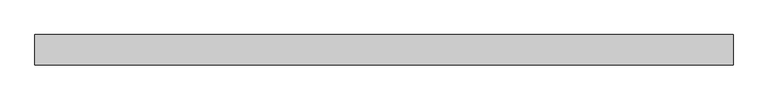
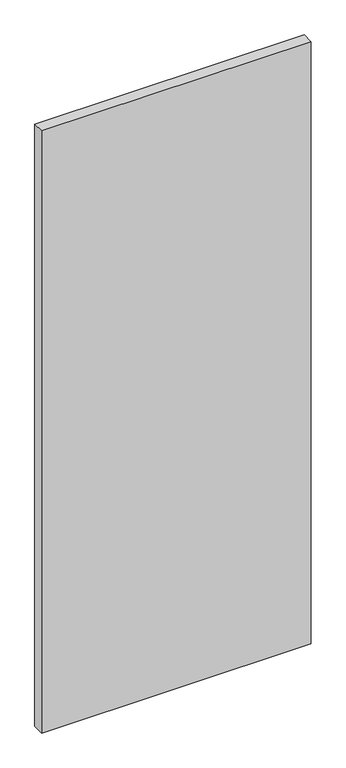
"""IFC4 building model written with IfcOpenShell, lengths in millimetres: proxy geometry, Generic Models 7:Generic Models 1:337419:Generic Models 1:337419 : Generic Models 7:Generic Models 1:337419:50 : Generic Models 7:Generic Models 1:337419:Generic Models 1:337419 : Generic Models 7:Generic Models 1:337419:301336."""

from ifc_helpers import new_model, si_unit, frame, origin, place, context, project, spatial, polyline, outline, extrude, source, transform, mapped, element, save


def generic_models_bfdba70c(model_context):
    return source(origin(), model_context, "Body", "SweptSolid", [
        extrude(outline(polyline([(593738.3225141, -536559.6725858), (593738.3225141, -536604.1225858), (592715.7367242, -536604.1225858), (592715.7367242, -536559.6725858), (593738.3225141, -536559.6725858)])), frame((0.0, 0.0, 22.0396518), z_axis=(0.0, 0.0, 1.0), x_axis=(1.0, 0.0, 0.0)), (0.0, 0.0, 1.0), 2413.3468131),
    ])


if __name__ == "__main__":
    model = new_model("IFC4")
    model_context = context("Model", 3, world=origin())
    ifc_project = project(units=[si_unit("LENGTHUNIT", "METRE", prefix="MILLI")], contexts=[model_context])
    site = spatial("IfcSite", under=ifc_project)
    building = spatial("IfcBuilding", under=site)
    placement = place(None, origin())
    generic_models_shape = generic_models_bfdba70c(model_context)
    element("IfcBuildingElementProxy", 1, Name="Generic Models 7:Generic Models 1:337419:Generic Models 1:337419 : Generic Models 7:Generic Models 1:337419:50 : Generic Models 7:Generic Models 1:337419:Generic Models 1:337419 : Generic Models 7:Generic Models 1:337419:301336", ObjectType="Generic Models 7:Generic Models 1:337419:Generic Models 1:337419 : Generic Models 7:Generic Models 1:337419:50 : Generic Models 7:Generic Models 1:337419:Generic Models 1:337419 : Generic Models 7:Generic Models 1:337419:301336", at=placement, inside=building, context=model_context, shape_type="MappedRepresentation", body=[
        mapped(generic_models_shape, transform((0.0, 0.0, 0.0), x_axis=(1.0, 0.0, 0.0), y_axis=(0.0, 1.0, 0.0), z_axis=(0.0, 0.0, 1.0))),
    ])
    save(model, "model.ifc")

# Revit data of these elements
# Type "Generic Models 7:Generic Models 1:337419:Generic Models 1:337419 : Generic Models 7:Generic Models 1:337419:50 : Generic Models 7:Generic Models 1:337419:Generic Models 1:337419 : Generic Models 7:Generic Models 1:337419:301336"
#   NameOverride = "Generic Models 7:Generic Models 1:337419:Generic Models 1:337419 : Generic Models 7:Generic Models 1:337419:301336"
#   ObjectTypeOverride = "Generic Models 1:337419 : Generic Models 7:Generic Models 1:337419"
#   Reference = "Generic Models 1"
#   Tag = "301336"
# Element 1 (IfcBuildingElementProxy, "Generic Models 7:Generic Models 1:337419:Generic Models 1:337419 : Generic Models 7:Generic Models 1:337419:50 : Generic Models 7:Generic Models 1:337419:Generic Models 1:337419 : Generic Models 7:Generic Models 1:337419:301336")
#   Materials on its faces: "METAL DOOR - SEE DOOR SCHEDULE"
# Materials
#   "METAL DOOR - SEE DOOR SCHEDULE": class "Unassigned", colour RGB 210 209 208, transparency 0, Keynote = "M05121300.02", Cost = 0
